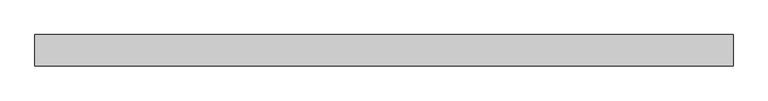
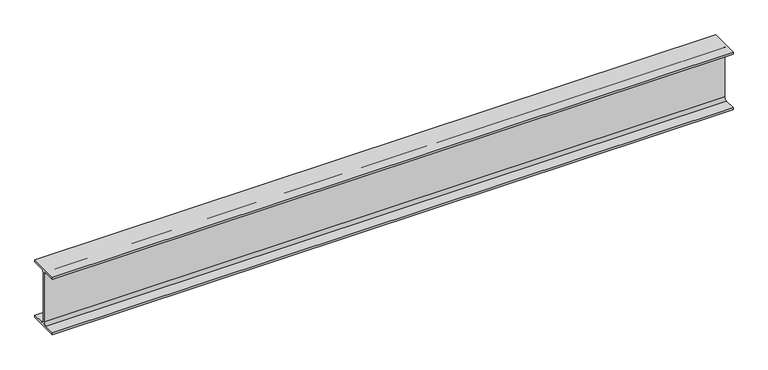
"""IFC4 building model written with IfcOpenShell, lengths in millimetres: beam geometry, 0912_Steel Framing_H-KSD3502 : H_SB_ASB_H-250x125x6x9."""

import ifcopenshell
import ifcopenshell.guid

model = None  # the IFC model being written
_history = None  # IfcOwnerHistory: only IFC2X3 demands one
_inside = {}  # id of a spatial element -> (the spatial element, [elements in it])
_under = {}  # id of a project, library or spatial element -> (it, [spatial elements below it])
_declared = {}  # id of a project -> (the project, [libraries it declares])
_typed = {}  # id of a type object -> (the type object, [elements of that type])
_made_of = {}  # id of a material, layer set ... -> (it, [elements and type objects made of it])


def new_model(schema):
    """Start an empty IFC model of exactly this schema.

    Asked for "IFC4X3", IfcOpenShell would pick the latest addendum, in which some entities
    have other attributes; the version numbers below select the first issue.
    IFC2X3 requires an IfcOwnerHistory on every rooted entity: one is made here for all.
    """
    global model, _history
    if schema == "IFC4X3":
        model = ifcopenshell.file(schema_version=(4, 3, 0, 0))
    else:
        model = ifcopenshell.file(schema=schema)
    _inside.clear()
    _under.clear()
    _declared.clear()
    _typed.clear()
    _made_of.clear()
    _history = None
    if model.schema == "IFC2X3":
        org = make("IfcOrganization", Name="unknown")
        user = make(
            "IfcPersonAndOrganization",
            ThePerson=make("IfcPerson", FamilyName="unknown"),
            TheOrganization=org,
        )
        app = make(
            "IfcApplication",
            ApplicationDeveloper=org,
            Version="unknown",
            ApplicationFullName="unknown",
            ApplicationIdentifier="unknown",
        )
        _history = make(
            "IfcOwnerHistory",
            OwningUser=user,
            OwningApplication=app,
            ChangeAction="ADDED",
            CreationDate=0,
        )
    return model


def make(cls, **values):
    """One entity of the class cls with the attributes given. An attribute that is None is left unset."""
    return model.create_entity(
        cls, **{name: value for name, value in values.items() if value is not None}
    )


def rooted(cls, **values):
    """An entity with a GlobalId (a new one), such as an element, a storey or a relation."""
    return make(cls, GlobalId=ifcopenshell.guid.new(), OwnerHistory=_history, **values)


def si_unit(unit_type, name, prefix=None):
    """IfcSIUnit, for example si_unit("LENGTHUNIT", "METRE", prefix="MILLI")."""
    return make("IfcSIUnit", UnitType=unit_type, Prefix=prefix, Name=name)


def assignment(units):
    """IfcUnitAssignment: the units of a project."""
    return None if units is None else make("IfcUnitAssignment", Units=units)


def point(xyz):
    """IfcCartesianPoint."""
    return None if xyz is None else make("IfcCartesianPoint", Coordinates=xyz)


def direction(xyz):
    """IfcDirection."""
    return None if xyz is None else make("IfcDirection", DirectionRatios=xyz)


def frame(location, z_axis=None, x_axis=None):
    """IfcAxis2Placement3D, a coordinate frame: its origin and axes. An axis left out is left unset."""
    return make(
        "IfcAxis2Placement3D",
        Location=point(location),
        Axis=direction(z_axis),
        RefDirection=direction(x_axis),
    )


def frame_2d(location, x_axis=None):
    """IfcAxis2Placement2D, a coordinate frame in the plane: its origin and x axis."""
    return make(
        "IfcAxis2Placement2D", Location=point(location), RefDirection=direction(x_axis)
    )


def origin():
    """The frame at (0, 0, 0) with its axes left unset."""
    return frame((0.0, 0.0, 0.0))


def place(relative_to, where):
    """IfcLocalPlacement: puts the frame where relative to a parent placement (None: the world)."""
    return make(
        "IfcLocalPlacement", PlacementRelTo=relative_to, RelativePlacement=where
    )


def context(
    kind, dimensions, precision=None, world=None, true_north=None, identifier=None
):
    """IfcGeometricRepresentationContext, for example the 3D "Model" context."""
    return make(
        "IfcGeometricRepresentationContext",
        ContextIdentifier=identifier,
        ContextType=kind,
        CoordinateSpaceDimension=dimensions,
        Precision=precision,
        WorldCoordinateSystem=world,
        TrueNorth=true_north,
    )


def project(units=None, contexts=None):
    """IfcProject with its units and contexts."""
    return rooted(
        "IfcProject",
        Name="project",
        RepresentationContexts=contexts,
        UnitsInContext=assignment(units),
    )


def spatial(cls, under=None, at=None, **own):
    """A site, building, storey or space (cls), placed at a placement, below another one or the project."""
    s = rooted(cls, ObjectPlacement=at, **own)
    if under is not None:
        _under.setdefault(under.id(), (under, []))[1].append(s)
    return s


def polyline(points):
    """IfcPolyline through the points."""
    return make("IfcPolyline", Points=[point(p) for p in points])


def circle_curve(where, radius):
    """IfcCircle in the frame where."""
    return make("IfcCircle", Position=where, Radius=radius)


def trimmed(basis, trim1, trim2, sense, master):
    """IfcTrimmedCurve: the piece of a basis curve between two trims."""
    return make(
        "IfcTrimmedCurve",
        BasisCurve=basis,
        Trim1=trim1,
        Trim2=trim2,
        SenseAgreement=sense,
        MasterRepresentation=master,
    )


def segment(curve, same_sense, transition):
    """IfcCompositeCurveSegment."""
    return make(
        "IfcCompositeCurveSegment",
        Transition=transition,
        SameSense=same_sense,
        ParentCurve=curve,
    )


def composite_curve(segments, self_intersect=None):
    """IfcCompositeCurve: segments joined end to end."""
    return make("IfcCompositeCurve", Segments=segments, SelfIntersect=self_intersect)


def outline(outer, holes=None, kind="AREA"):
    """IfcArbitraryClosedProfileDef: a profile drawn as a closed curve; with holes, ...WithVoids."""
    if holes is None:
        return make("IfcArbitraryClosedProfileDef", ProfileType=kind, OuterCurve=outer)
    return make(
        "IfcArbitraryProfileDefWithVoids",
        ProfileType=kind,
        OuterCurve=outer,
        InnerCurves=holes,
    )


def extrude(swept, where, along, depth):
    """IfcExtrudedAreaSolid: the profile swept, set in the frame where, extruded along a direction by depth."""
    return make(
        "IfcExtrudedAreaSolid",
        SweptArea=swept,
        Position=where,
        ExtrudedDirection=direction(along),
        Depth=depth,
    )


def shape(context_of_items, identifier, shape_type, items):
    """IfcShapeRepresentation: the items that make up one representation, for example the "Body"."""
    return make(
        "IfcShapeRepresentation",
        ContextOfItems=context_of_items,
        RepresentationIdentifier=identifier,
        RepresentationType=shape_type,
        Items=items,
    )


def source(mapping_origin, context_of_items, identifier, shape_type, items):
    """IfcRepresentationMap: a shape defined once, which mapped items show again and again."""
    return make(
        "IfcRepresentationMap",
        MappingOrigin=mapping_origin,
        MappedRepresentation=shape(context_of_items, identifier, shape_type, items),
    )


def transform(
    local_origin,
    x_axis=None,
    y_axis=None,
    z_axis=None,
    scale=None,
    scale2=None,
    scale3=None,
    uniform=True,
):
    """IfcCartesianTransformationOperator3D, or its non-uniform kind. x_axis, y_axis, z_axis: its Axis1, 2, 3."""
    if uniform:
        return make(
            "IfcCartesianTransformationOperator3D",
            Axis1=direction(x_axis),
            Axis2=direction(y_axis),
            LocalOrigin=point(local_origin),
            Scale=scale,
            Axis3=direction(z_axis),
        )
    return make(
        "IfcCartesianTransformationOperator3DnonUniform",
        Axis1=direction(x_axis),
        Axis2=direction(y_axis),
        LocalOrigin=point(local_origin),
        Scale=scale,
        Axis3=direction(z_axis),
        Scale2=scale2,
        Scale3=scale3,
    )


def mapped(mapping_source, mapping_target):
    """IfcMappedItem: shows the shape of a source again, moved by a transform."""
    return make(
        "IfcMappedItem", MappingSource=mapping_source, MappingTarget=mapping_target
    )


def made_of(thing, what):
    """Note that an element or type object is made of a material, layer set ...; save() writes the relation."""
    if what is not None:
        _made_of.setdefault(what.id(), (what, []))[1].append(thing)
    return thing


def element(
    cls,
    number,
    at=None,
    inside=None,
    cuts=None,
    type_object=None,
    material=None,
    context=None,
    identifier="Body",
    shape_type=None,
    held_by="IfcProductDefinitionShape",
    body=None,
    shapes=None,
    **own,
):
    """One element of the class cls, such as IfcWall. Its Tag is "e" and its number.

    at: its placement. inside: the storey or other place that contains it. cuts: it is an
    opening in that element (IfcRelVoidsElement). A single representation is given by context,
    identifier, shape_type and body (its items); several are given by shapes. held_by: the class
    of the entity that holds the representations. save() writes the other relations.
    """
    e = rooted(cls, Tag="e%d" % number, ObjectPlacement=at, **own)
    if body is not None:
        shapes = [shape(context, identifier, shape_type, body)]
    if shapes is not None:
        e.Representation = make(held_by, Representations=shapes)
    if inside is not None:
        _inside.setdefault(inside.id(), (inside, []))[1].append(e)
    if cuts is not None:
        rooted(
            "IfcRelVoidsElement", RelatingBuildingElement=cuts, RelatedOpeningElement=e
        )
    if type_object is not None:
        _typed.setdefault(type_object.id(), (type_object, []))[1].append(e)
    return made_of(e, material)


def aggregate(whole, parts):
    """IfcRelAggregates: a whole, such as a stair, and the parts it consists of."""
    return rooted("IfcRelAggregates", RelatingObject=whole, RelatedObjects=parts)


def save(model, path):
    """Write the relations noted so far, then the file.

    IfcRelAggregates (storeys below a building ...), IfcRelContainedInSpatialStructure (elements
    in a storey), IfcRelDefinesByType, IfcRelAssociatesMaterial and IfcRelDeclares: one each for
    every whole, place, type object, material and project.
    """
    for whole, parts in _under.values():
        aggregate(whole, parts)
    for where, things in _inside.values():
        rooted(
            "IfcRelContainedInSpatialStructure",
            RelatedElements=things,
            RelatingStructure=where,
        )
    for kind, things in _typed.values():
        rooted("IfcRelDefinesByType", RelatedObjects=things, RelatingType=kind)
    for what, things in _made_of.values():
        rooted("IfcRelAssociatesMaterial", RelatedObjects=things, RelatingMaterial=what)
    for by, libraries in _declared.values():
        rooted("IfcRelDeclares", RelatingContext=by, RelatedDefinitions=libraries)
    model.write(path)


def beam_8986b571(model_context):
    return source(origin(), model_context, "Body", "SweptSolid", [
        extrude(outline(composite_curve([segment(polyline([(62.5, -116.0), (62.5, -125.0), (-62.5, -125.0), (-62.5, -116.0), (-15.0, -116.0)]), True, "CONTINUOUS"), segment(trimmed(circle_curve(frame_2d((-15.0, -104.0)), 12.0), [point((-15.0, -116.0))], [point((-3.0, -104.0))], True, "CARTESIAN"), True, "CONTINUOUS"), segment(polyline([(-3.0, -104.0), (-3.0, 104.0)]), True, "CONTINUOUS"), segment(trimmed(circle_curve(frame_2d((-15.0, 104.0)), 12.0), [point((-3.0, 104.0))], [point((-15.0, 116.0))], True, "CARTESIAN"), True, "CONTINUOUS"), segment(polyline([(-15.0, 116.0), (-62.5, 116.0), (-62.5, 125.0), (62.5, 125.0), (62.5, 116.0), (15.0, 116.0)]), True, "CONTINUOUS"), segment(trimmed(circle_curve(frame_2d((15.0, 104.0)), 12.0), [point((15.0, 116.0))], [point((3.0, 104.0))], True, "CARTESIAN"), True, "CONTINUOUS"), segment(polyline([(3.0, 104.0), (3.0, -104.0)]), True, "CONTINUOUS"), segment(trimmed(circle_curve(frame_2d((15.0, -104.0)), 12.0), [point((3.0, -104.0))], [point((15.0, -116.0))], True, "CARTESIAN"), True, "CONTINUOUS"), segment(polyline([(15.0, -116.0), (62.5, -116.0)]), True, "CONTINUOUS")], self_intersect=False)), frame((-1382.3488581, 0.0, 0.0), z_axis=(1.0, 0.0, 0.0), x_axis=(0.0, 1.0, 0.0)), (0.0, 0.0, 1.0), 2794.6488581),
    ])


if __name__ == "__main__":
    model = new_model("IFC4")
    model_context = context("Model", 3, world=origin())
    ifc_project = project(units=[si_unit("LENGTHUNIT", "METRE", prefix="MILLI")], contexts=[model_context])
    site = spatial("IfcSite", under=ifc_project)
    building = spatial("IfcBuilding", under=site)
    placement = place(None, origin())
    beam_shape = beam_8986b571(model_context)
    element("IfcBeam", 1, ObjectType="0912_Steel Framing_H-KSD3502 : H_SB_ASB_H-250x125x6x9", at=placement, inside=building, context=model_context, shape_type="MappedRepresentation", body=[
        mapped(beam_shape, transform((0.0, 0.0, 0.0), x_axis=(1.0, 0.0, 0.0), y_axis=(0.0, 1.0, 0.0), z_axis=(0.0, 0.0, 1.0))),
    ])
    save(model, "model.ifc")

# Revit data of these elements
# Type "0912_Steel Framing_H-KSD3502 : H_SB_ASB_H-250x125x6x9"
#   H_WM Code_1 = "S01AA003-00001 | Main Steel Structure Fabrication Work | Shelter/Building | Light Steel - Standard (30KG/M>Weight) | Material: (   )"
#   H_WM Code_2 = "S03AA029-00001 | Main Steel Structure Erection Work | Shelter/Building | Light Steel (30KG/M>Weight) | Material: (   )"
#   H_WM Code_3 = "S01AA010-00001 | Main Steel Structure Fabrication Work | Shelter/Building | Steel Painting/Coating | for Non-Fireproofed Steel Surface, Surface Preparation, Primer, Second & Final Coat | Material: (   )"
#   H_Q'ty Cal Type Tag = "SB-Q2"
#   Width = 12.5 cm
#   Web Thickness = 0.6 cm
#   Web Fillet = 1.2 cm
#   Warping Constant = 42539.8 cm⁶
#   W = 0
#   Torsional Moment of Inertia = 7.8102 cm⁴
#   Section Area = 37.66 cm²
#   Plastic Modulus weak axis = 73.1 cm³
#   Plastic Modulus strong axis = 366.0 cm³
#   Perimeter = 0.97 m²/m
#   Nominal Weight = 29.60 kgf/m
#   Moment of Inertia weak axis = 294.00 cm⁴
#   Moment of Inertia strong axis = 4050.00 cm⁴
#   Height = 25.0 cm
#   Flange Thickness = 0.9 cm
#   Elastic Modulus weak axis = 47.0 cm³
#   Elastic Modulus strong axis = 324.0 cm³
#   Centroid Vertical = 12.5 cm
#   Centroid Horizontal = 6.25 cm
#   Ix = 40500000
#   Length [instance default] = 1.5240 m
#   Zx = 366000
#   b = 0.1250 m
#   h = 0.2500 m
#   r = 0.0120 m
#   s = 0.0060 m
#   t = 0.0090 m
#   A = 0.003766 m²
#   Structural Material [instance default] = Steel, 45-345
#   Assembly Code = ""
# Element 1 (IfcBeam, "0912_Steel Framing_H-KSD3502 : H_SB_ASB_H-250x125x6x9")
#   Structural Material = none
# Materials
#   "Steel, 45-345": class "Metal", colour RGB 189 187 185, transparency 0, Description = "Steel 345 MPa", Cost = 0
